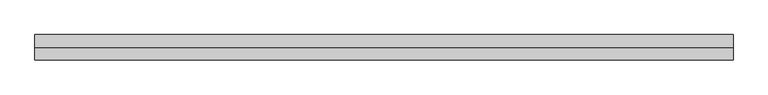
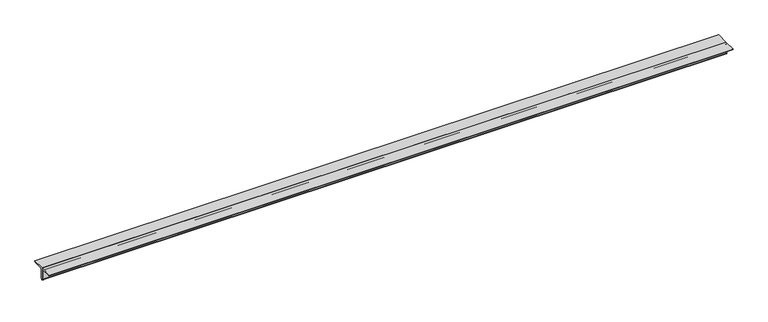
"""IFC4 building model written with IfcOpenShell, lengths in millimetres: member geometry, 0123_Steel Framing_2Ls-KSD3502 : H_SB_AR_S04_2Ls-130x130x12_VBR2."""

from ifc_helpers import new_model, si_unit, point, frame, frame_2d, origin, place, context, project, spatial, polyline, circle_curve, trimmed, segment, composite_curve, outline, extrude, source, transform, mapped, element, save


def member_9327e08a(model_context):
    return source(origin(), model_context, "Body", "SweptSolid", [
        extrude(outline(composite_curve([segment(polyline([(0.0, 36.4), (130.0, 36.4)]), True, "CONTINUOUS"), segment(trimmed(circle_curve(frame_2d((118.0, 36.4)), 12.0), [point((130.0, 36.4))], [point((118.0, 24.4))], False, "CARTESIAN"), True, "CONTINUOUS"), segment(polyline([(118.0, 24.4), (24.0, 24.4)]), True, "CONTINUOUS"), segment(trimmed(circle_curve(frame_2d((24.0, 12.4)), 12.0), [point((24.0, 24.4))], [point((12.0, 12.4))], True, "CARTESIAN"), True, "CONTINUOUS"), segment(polyline([(12.0, 12.4), (12.0, -81.6)]), True, "CONTINUOUS"), segment(trimmed(circle_curve(frame_2d((0.0, -81.6)), 12.0), [point((12.0, -81.6))], [point((0.0, -93.6))], False, "CARTESIAN"), True, "CONTINUOUS"), segment(polyline([(0.0, -93.6), (0.0, 36.4)]), True, "CONTINUOUS")], self_intersect=False)), frame((-3534.7173983, 0.0, 0.0), z_axis=(1.0, 0.0, 0.0), x_axis=(0.0, 1.0, 0.0)), (0.0, 0.0, 1.0), 7187.6786398),
        extrude(outline(composite_curve([segment(polyline([(0.0, 36.4), (0.0, -93.6)]), True, "CONTINUOUS"), segment(trimmed(circle_curve(frame_2d((0.0, -81.6)), 12.0), [point((0.0, -93.6))], [point((-12.0, -81.6))], False, "CARTESIAN"), True, "CONTINUOUS"), segment(polyline([(-12.0, -81.6), (-12.0, 12.4)]), True, "CONTINUOUS"), segment(trimmed(circle_curve(frame_2d((-24.0, 12.4)), 12.0), [point((-12.0, 12.4))], [point((-24.0, 24.4))], True, "CARTESIAN"), True, "CONTINUOUS"), segment(polyline([(-24.0, 24.4), (-118.0, 24.4)]), True, "CONTINUOUS"), segment(trimmed(circle_curve(frame_2d((-118.0, 36.4)), 12.0), [point((-118.0, 24.4))], [point((-130.0, 36.4))], False, "CARTESIAN"), True, "CONTINUOUS"), segment(polyline([(-130.0, 36.4), (0.0, 36.4)]), True, "CONTINUOUS")], self_intersect=False)), frame((-3534.7173983, 0.0, 0.0), z_axis=(1.0, 0.0, 0.0), x_axis=(0.0, 1.0, 0.0)), (0.0, 0.0, 1.0), 7187.6786398),
    ])


if __name__ == "__main__":
    model = new_model("IFC4")
    model_context = context("Model", 3, world=origin())
    ifc_project = project(units=[si_unit("LENGTHUNIT", "METRE", prefix="MILLI")], contexts=[model_context])
    site = spatial("IfcSite", under=ifc_project)
    building = spatial("IfcBuilding", under=site)
    placement = place(None, origin())
    member_shape = member_9327e08a(model_context)
    element("IfcMember", 1, ObjectType="0123_Steel Framing_2Ls-KSD3502 : H_SB_AR_S04_2Ls-130x130x12_VBR2", at=placement, inside=building, context=model_context, shape_type="MappedRepresentation", body=[
        mapped(member_shape, transform((0.0, 0.0, 0.0), x_axis=(1.0, 0.0, 0.0), y_axis=(0.0, 1.0, 0.0), z_axis=(0.0, 0.0, 1.0))),
    ])
    save(model, "model.ifc")

# Revit data of these elements
# Type "0123_Steel Framing_2Ls-KSD3502 : H_SB_AR_S04_2Ls-130x130x12_VBR2"
#   Assembly Code = "B10"
#   Legs = "SLBB"
#   W = 8.97
#   Perimeter = 1.04 m²/m
#   Nominal Weight = 46.80 kgf/m
#   Length [instance default] = 1000 mm
#   Space = 0 mm
#   b = 130 mm
#   d = 130 mm
#   t = 12 mm
#   y = 36.4 mm
#   A = 0.005952 m²
#   Structural Material [instance default] = Steel ASTM A36
# Element 1 (IfcMember, "0123_Steel Framing_2Ls-KSD3502 : H_SB_AR_S04_2Ls-130x130x12_VBR2")
#   Structural Material = Steel, 45-345
#   Materials on its faces: "Steel, 45-345"
# Materials
#   "Steel ASTM A36": class "Metal", colour RGB 199 199 199, transparency 0, Description = "Structural steel, ASTM A36 Grade B, mill finish", Cost = 0
#   "Steel, 45-345": class "Metal", colour RGB 189 187 185, transparency 0, Description = "Steel 345 MPa", Cost = 0
